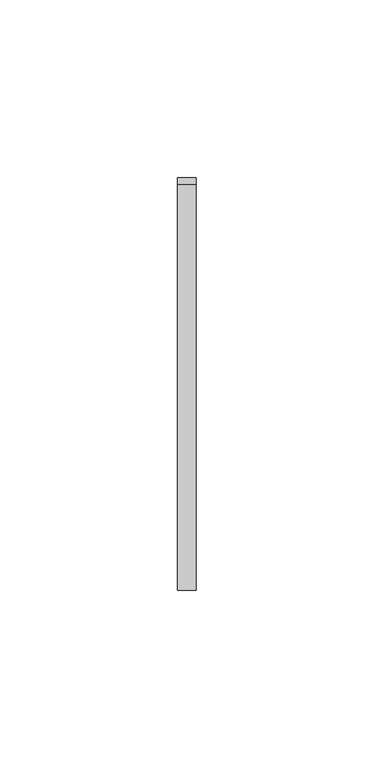
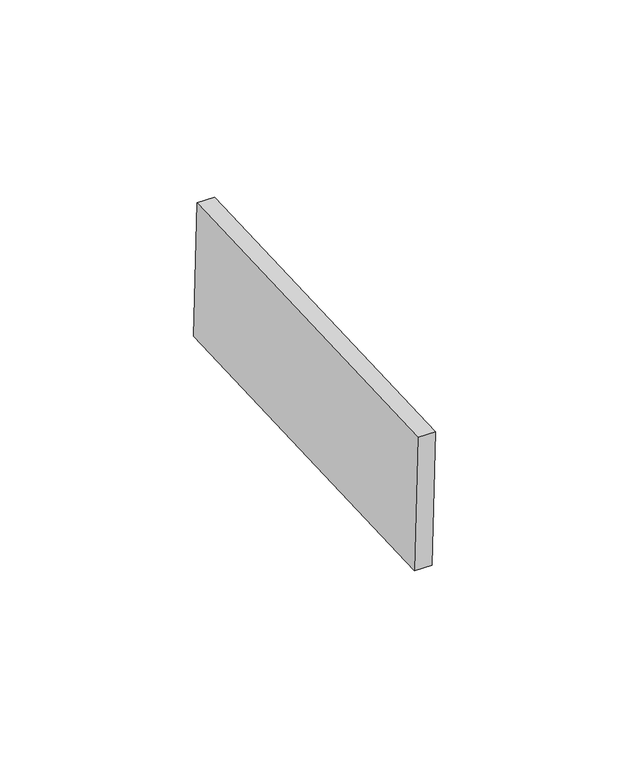
"""IFC4 building model written with IfcOpenShell, lengths in millimetres: proxy geometry, Inner panel:Inner panel:1:Inner panel:1 : Inner panel:Inner panel:300324:2:Inner panel:1:Inner panel:1 : Inner panel:Inner panel:300324:2 : Inner panel:Inner panel:1:Inner panel:1 : Inner panel:Inner panel:300324:300043:60 : Inner panel:Inner panel:1:Inner panel:1 : Inner panel:Inner panel:300324:2:Inner panel:1:Inner panel:1 : Inner panel:Inner panel:300324:2 : Inner panel:Inner panel:1:Inner panel:1 : Inner panel:Inner panel:300324:300043:308120."""

from ifc_helpers import new_model, si_unit, frame, origin, place, context, project, spatial, polyline, outline, extrude, source, transform, mapped, element, save


def generic_models_97b75c92(model_context):
    return source(origin(), model_context, "Body", "SweptSolid", [
        extrude(outline(polyline([(0.0, -114.3), (0.0, 0.0), (5.2138089, 0.0), (5.2138089, -114.3), (0.0, -114.3)])), frame((593530.195117, -579007.2622385, 3952.103089), z_axis=(0.0, -0.04163054471216399, 0.9991330730923527), x_axis=(-1.0, 0.0, 0.0)), (0.0, 0.0, 1.0), 43.2233908),
    ])


if __name__ == "__main__":
    model = new_model("IFC4")
    model_context = context("Model", 3, world=origin())
    ifc_project = project(units=[si_unit("LENGTHUNIT", "METRE", prefix="MILLI")], contexts=[model_context])
    site = spatial("IfcSite", under=ifc_project)
    building = spatial("IfcBuilding", under=site)
    placement = place(None, origin())
    generic_models_shape = generic_models_97b75c92(model_context)
    element("IfcBuildingElementProxy", 1, Name="Inner panel:Inner panel:1:Inner panel:1 : Inner panel:Inner panel:300324:2:Inner panel:1:Inner panel:1 : Inner panel:Inner panel:300324:2 : Inner panel:Inner panel:1:Inner panel:1 : Inner panel:Inner panel:300324:300043:60 : Inner panel:Inner panel:1:Inner panel:1 : Inner panel:Inner panel:300324:2:Inner panel:1:Inner panel:1 : Inner panel:Inner panel:300324:2 : Inner panel:Inner panel:1:Inner panel:1 : Inner panel:Inner panel:300324:300043:308120", ObjectType="Inner panel:Inner panel:1:Inner panel:1 : Inner panel:Inner panel:300324:2:Inner panel:1:Inner panel:1 : Inner panel:Inner panel:300324:2 : Inner panel:Inner panel:1:Inner panel:1 : Inner panel:Inner panel:300324:300043:60 : Inner panel:Inner panel:1:Inner panel:1 : Inner panel:Inner panel:300324:2:Inner panel:1:Inner panel:1 : Inner panel:Inner panel:300324:2 : Inner panel:Inner panel:1:Inner panel:1 : Inner panel:Inner panel:300324:300043:308120", at=placement, inside=building, context=model_context, shape_type="MappedRepresentation", body=[
        mapped(generic_models_shape, transform((0.0, 0.0, 0.0), x_axis=(1.0, 0.0, 0.0), y_axis=(0.0, 1.0, 0.0), z_axis=(0.0, 0.0, 1.0))),
    ])
    save(model, "model.ifc")

# Revit data of these elements
# Type "Inner panel:Inner panel:1:Inner panel:1 : Inner panel:Inner panel:300324:2:Inner panel:1:Inner panel:1 : Inner panel:Inner panel:300324:2 : Inner panel:Inner panel:1:Inner panel:1 : Inner panel:Inner panel:300324:300043:60 : Inner panel:Inner panel:1:Inner panel:1 : Inner panel:Inner panel:300324:2:Inner panel:1:Inner panel:1 : Inner panel:Inner panel:300324:2 : Inner panel:Inner panel:1:Inner panel:1 : Inner panel:Inner panel:300324:300043:308120"
#   NameOverride = "Inner panel:Inner panel:1:Inner panel:1 : Inner panel:Inner panel:300324:2:Inner panel:1:Inner panel:1 : Inner panel:Inner panel:300324:2 : Inner panel:Inner panel:1:Inner panel:1 : Inner panel:Inner panel:300324:300043:308120"
#   ObjectTypeOverride = "Inner panel:1:Inner panel:1 : Inner panel:Inner panel:300324:2 : Inner panel:Inner panel:1:Inner panel:1 : Inner panel:Inner panel:300324:300043"
#   Reference = "Inner panel"
#   Tag = "308120"
# Element 1 (IfcBuildingElementProxy, "Inner panel:Inner panel:1:Inner panel:1 : Inner panel:Inner panel:300324:2:Inner panel:1:Inner panel:1 : Inner panel:Inner panel:300324:2 : Inner panel:Inner panel:1:Inner panel:1 : Inner panel:Inner panel:300324:300043:60 : Inner panel:Inner panel:1:Inner panel:1 : Inner panel:Inner panel:300324:2:Inner panel:1:Inner panel:1 : Inner panel:Inner panel:300324:2 : Inner panel:Inner panel:1:Inner panel:1 : Inner panel:Inner panel:300324:300043:308120")
#   Materials on its faces: "SLIDING CLIP"
# Materials
#   "SLIDING CLIP": class "Generic", colour RGB 120 120 120, transparency 0, Cost = 0
